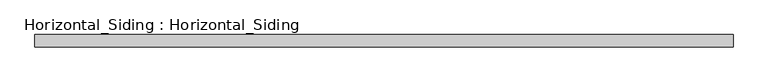
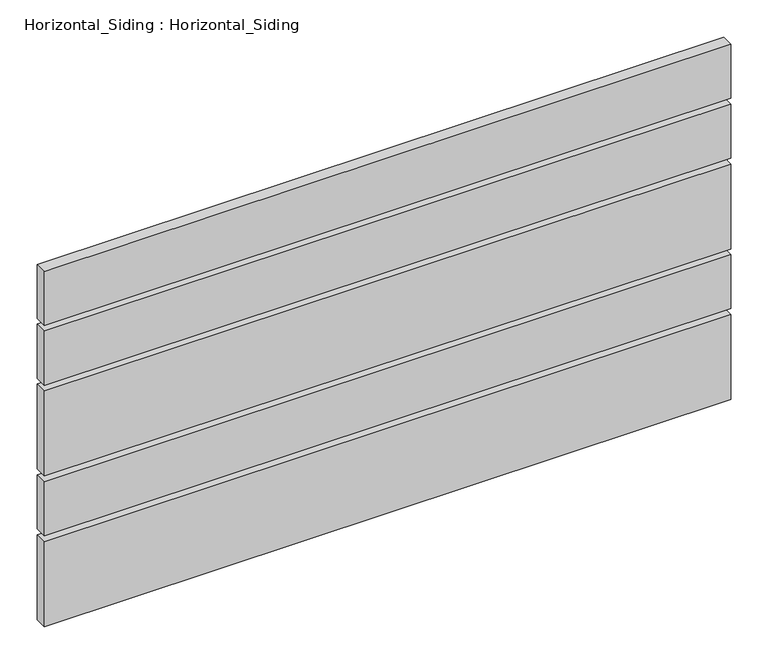
"""IFC4 building model written with IfcOpenShell, lengths in millimetres: plate geometry, Horizontal_Siding : Horizontal_Siding."""

from ifc_helpers import new_model, si_unit, frame, origin, place, context, project, spatial, polyline, outline, extrude, source, transform, mapped, element, save


def horizontal_siding_horizontal_siding_6226d231(model_context):
    return source(origin(), model_context, "Body", "SweptSolid", [
        extrude(outline(polyline([(533.4, -19.05), (-533.4, -19.05), (-533.4, 0.0), (533.4, 0.0), (533.4, -19.05)])), frame((0.0, 0.0, 9.525), z_axis=(0.0, 0.0, 1.0), x_axis=(1.0, 0.0, 0.0)), (0.0, 0.0, 1.0), 139.7),
        extrude(outline(polyline([(533.4, -19.05), (-533.4, -19.05), (-533.4, 0.0), (533.4, 0.0), (533.4, -19.05)])), frame((0.0, 0.0, 158.75), z_axis=(0.0, 0.0, 1.0), x_axis=(1.0, 0.0, 0.0)), (0.0, 0.0, 1.0), 88.9),
        extrude(outline(polyline([(533.4, -19.05), (-533.4, -19.05), (-533.4, 0.0), (533.4, 0.0), (533.4, -19.05)])), frame((0.0, 0.0, 257.175), z_axis=(0.0, 0.0, 1.0), x_axis=(1.0, 0.0, 0.0)), (0.0, 0.0, 1.0), 139.7),
        extrude(outline(polyline([(533.4, -19.05), (-533.4, -19.05), (-533.4, 0.0), (533.4, 0.0), (533.4, -19.05)])), frame((0.0, 0.0, 406.4), z_axis=(0.0, 0.0, 1.0), x_axis=(1.0, 0.0, 0.0)), (0.0, 0.0, 1.0), 88.9),
        extrude(outline(polyline([(533.4, -19.05), (-533.4, -19.05), (-533.4, 0.0), (533.4, 0.0), (533.4, -19.05)])), frame((0.0, 0.0, 504.825), z_axis=(0.0, 0.0, 1.0), x_axis=(1.0, 0.0, 0.0)), (0.0, 0.0, 1.0), 88.9),
    ])


if __name__ == "__main__":
    model = new_model("IFC4")
    model_context = context("Model", 3, world=origin())
    ifc_project = project(units=[si_unit("LENGTHUNIT", "METRE", prefix="MILLI")], contexts=[model_context])
    site = spatial("IfcSite", under=ifc_project)
    building = spatial("IfcBuilding", under=site)
    placement = place(None, origin())
    horizontal_siding_horizontal_siding_shape = horizontal_siding_horizontal_siding_6226d231(model_context)
    element("IfcPlate", 1, ObjectType="Horizontal_Siding : Horizontal_Siding", at=placement, inside=building, context=model_context, shape_type="MappedRepresentation", body=[
        mapped(horizontal_siding_horizontal_siding_shape, transform((0.0, 0.0, 0.0), x_axis=(1.0, 0.0, 0.0), y_axis=(0.0, 1.0, 0.0), z_axis=(0.0, 0.0, 1.0))),
    ])
    save(model, "model.ifc")

# Revit data of these elements
# Type "Horizontal_Siding : Horizontal_Siding"
#   Type Mark = "OUT"
#   Analytic Construction = "<None>"
#   extend = 0' - 2 3/4"
#   Width_2 = 0' - 3 1/2"
#   Width_1 = 0' - 5 1/2"
#   Gap = 0' - 0 3/8"
#   Plank Material = SLOTTED WOOD FENCE (THERMALLY MODIFIED WOOD: ARBOR WOOD)\n(EXTERIOR STAIN : PENOFIN VERDE EXT. STAIN - COLOR: CEDAR)
# Element 1 (IfcPlate, "Horizontal_Siding : Horizontal_Siding")
#   Materials on its faces: "SLOTTED WOOD FENCE (THERMALLY MODIFIED WOOD: ARBOR WOOD)\n(EXTERIOR STAIN : PENOFIN VERDE EXT. STAIN - COLOR: CEDAR)"
# Materials
#   "SLOTTED WOOD FENCE (THERMALLY MODIFIED WOOD: ARBOR WOOD)\n(EXTERIOR STAIN : PENOFIN VERDE EXT. STAIN - COLOR: CEDAR)": class "Wood", colour RGB 164 134 123, transparency 0, Description = "Pinus Echinata", Cost = 0
